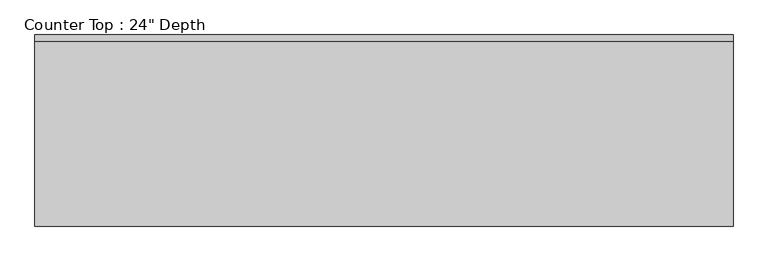
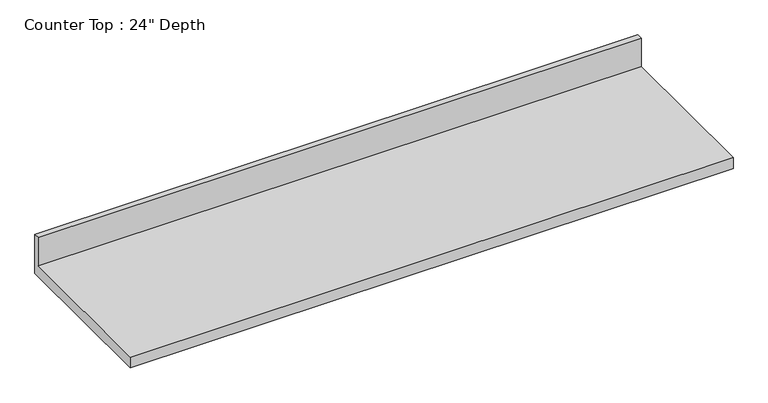
"""IFC4 building model written with IfcOpenShell, lengths in millimetres: furniture geometry."""

from ifc_helpers import new_model, si_unit, frame, origin, place, context, project, spatial, polyline, outline, extrude, source, transform, mapped, element, save


def furniture_ef5f263e(model_context):
    return source(origin(), model_context, "Body", "SweptSolid", [
        extrude(outline(polyline([(0.0, 1016.0), (0.0, 876.3), (-558.8, 876.3), (-558.8, 914.4), (-19.05, 914.4), (-19.05, 1016.0), (0.0, 1016.0)])), frame((-1200.4622951, 0.0, 0.0), z_axis=(1.0, 0.0, 0.0), x_axis=(0.0, 1.0, 0.0)), (0.0, 0.0, 1.0), 2041.525),
    ])


if __name__ == "__main__":
    model = new_model("IFC4")
    model_context = context("Model", 3, world=origin())
    ifc_project = project(units=[si_unit("LENGTHUNIT", "METRE", prefix="MILLI")], contexts=[model_context])
    site = spatial("IfcSite", under=ifc_project)
    building = spatial("IfcBuilding", under=site)
    placement = place(None, origin())
    furniture_shape = furniture_ef5f263e(model_context)
    element("IfcFurniture", 1, ObjectType="Counter Top : 24\" Depth", at=placement, inside=building, context=model_context, shape_type="MappedRepresentation", body=[
        mapped(furniture_shape, transform((0.0, 0.0, 0.0), x_axis=(1.0, 0.0, 0.0), y_axis=(0.0, 1.0, 0.0), z_axis=(0.0, 0.0, 1.0))),
    ])
    save(model, "model.ifc")

# Revit data of these elements
# Type "Counter Top : 24\" Depth"
#   Keynote = "M12366116.01"
#   Assembly Code = "C1030400"
#   Counter Thickness = 0' - 1 1/2"
#   Depth = 1' - 10"
#   Height = 3' - 0"
#   Length [instance default] = 8' - 0"
#   Counter Top Material = none
# Element 1 (IfcFurniture, "Counter Top : 24\" Depth")
#   Length = 6' - 8 3/8"
